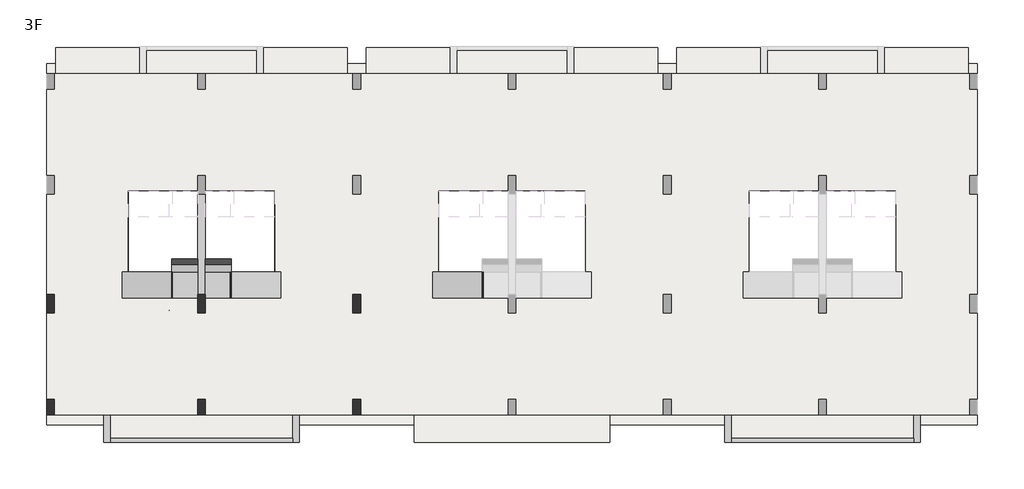
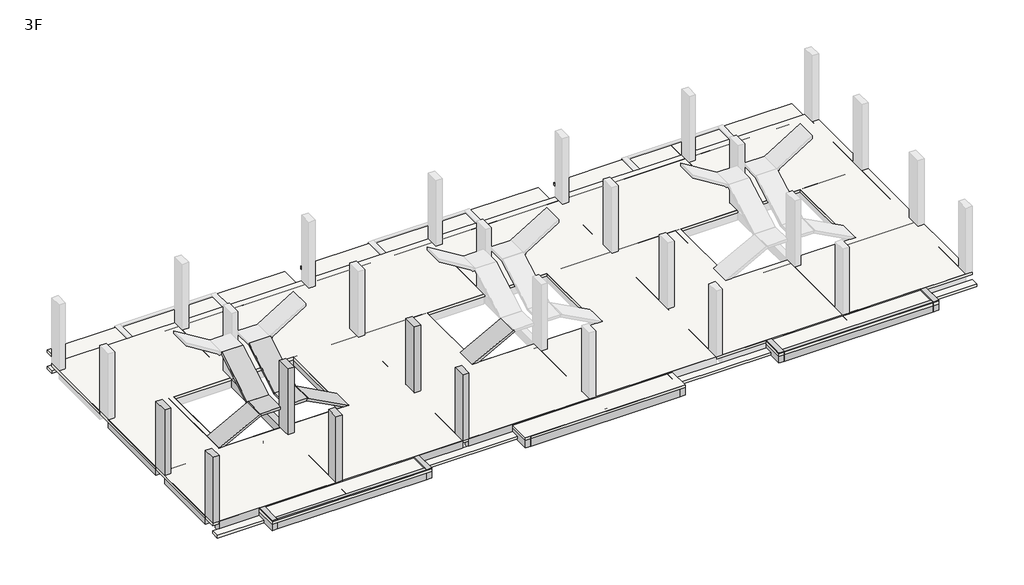
# One storey, part 1 of 3: 33 beams, 6 columns, 3 slabs.
"""IFC4 building model written with IfcOpenShell, lengths in millimetres."""

from ifc_helpers import new_model, si_unit, frame, origin, place, context, project, spatial, polyline, outline, extrude, faceted_brep, element, save

model = new_model("IFC4")

# Units and contexts
model_context = context("Model", 3, world=origin())
ifc_project = project(units=[si_unit("LENGTHUNIT", "METRE", prefix="MILLI")], contexts=[model_context])

# Site, building, storey
site = spatial("IfcSite", under=ifc_project)
building = spatial("IfcBuilding", under=site)
storey = spatial("IfcBuildingStorey", under=building, Name="3F", Elevation=7330.0)

# Beams
placement = place(None, origin())
element("IfcBeam", 1, ObjectType="M_Concrete-Rectangular Beam : 1000x120", at=placement, inside=storey, context=model_context, shape_type="Brep", body=[
    faceted_brep([(4730.4772067, 5424.9999998, 8380.0), (4730.4772067, 4424.9999998, 8380.0), (4787.1330577, 4424.9999998, 8274.2166623), (4787.1330577, 5424.9999998, 8274.2166623), (4700.0000007, 5424.9999998, 8363.6768996), (2770.0, 5424.9999998, 7330.0), (2770.0, 4424.9999998, 7330.0), (4700.0000007, 4424.9999998, 8363.6768996), (3024.1661582, 4424.9999998, 7330.0), (4760.5888269, 4424.9999998, 8260.0), (3024.1661582, 4449.9999998, 7330.0), (3020.0, 4449.9999998, 7327.7686728), (3020.0, 5424.9999998, 7327.7686728), (4760.5888269, 5424.9999998, 8260.0), (3020.0, 5424.9999998, 7330.0), (3020.0, 4449.9999998, 7330.0)], [[[0, 1, 2, 3]], [[1, 0, 4, 5, 6, 7]], [[2, 1, 7, 6, 8, 9]], [[3, 2, 9, 8, 10, 11, 12, 13]], [[0, 3, 13, 12, 14, 5, 4]], [[5, 14, 15, 10, 8, 6]], [[14, 12, 11, 15]], [[10, 15, 11]]]),
])
element("IfcBeam", 2, ObjectType="M_Concrete-Rectangular Beam : 1000x120", at=placement, inside=storey, context=model_context, shape_type="Brep", body=[
    faceted_brep([(4700.0000007, 7550.0000002, 9580.0), (5700.0000007, 7550.0000002, 9580.0), (5700.0000007, 7609.0063595, 9475.5095719), (4700.0000007, 7609.0063595, 9475.5095719), (4700.0000007, 5424.9999998, 8380.0), (4700.0000007, 5484.0063591, 8275.5095719), (5700.0000007, 5484.0063591, 8275.5095719), (5700.0000007, 5424.9999998, 8380.0), (5700.0000007, 5524.9999998, 8298.6589219), (5700.0000007, 7581.5414925, 9460.0), (4700.0000007, 5524.9999998, 8298.6589219), (4700.0000007, 7581.5414925, 9460.0)], [[[0, 1, 2, 3]], [[4, 5, 6, 7]], [[1, 0, 4, 7]], [[2, 1, 7, 6, 8, 9]], [[3, 2, 9, 8, 6, 5, 10, 11]], [[0, 3, 11, 10, 5, 4]]]),
])
element("IfcBeam", 3, ObjectType="M_Concrete-Rectangular Beam : 1000x120", at=placement, inside=storey, context=model_context, shape_type="Brep", body=[
    faceted_brep([(5700.0000007, 5524.9999998, 8260.0), (4700.0000007, 5524.9999998, 8260.0), (4700.0000007, 5524.9999998, 8298.6589219), (5700.0000007, 5524.9999998, 8298.6589219), (5700.0000007, 4424.9999998, 8260.0), (5700.0000007, 4424.9999998, 8380.0), (4730.4772067, 4424.9999998, 8380.0), (4787.1330577, 4424.9999998, 8274.2166623), (4760.5888269, 4424.9999998, 8260.0), (5700.0000007, 5424.9999998, 8380.0), (4700.0000007, 5424.9999998, 8380.0), (4700.0000007, 4424.9999998, 8380.0), (5700.0000007, 5484.0063591, 8275.5095719), (4760.5888269, 5424.9999998, 8260.0), (4700.0000007, 5424.9999998, 8260.0), (4700.0000007, 4424.9999998, 8363.6768996), (4700.0000007, 5484.0063591, 8275.5095719), (4700.0000007, 5424.9999998, 8363.6768996), (4730.4772067, 5424.9999998, 8380.0), (4787.1330577, 5424.9999998, 8274.2166623)], [[[0, 1, 2, 3]], [[4, 5, 6, 7, 8]], [[6, 5, 9, 10, 11]], [[5, 4, 0, 3, 12, 9]], [[1, 0, 4, 8, 13, 14]], [[15, 11, 10, 16, 2, 1, 14, 17]], [[6, 18, 19, 7]], [[18, 6, 15, 17]], [[7, 19, 13, 8]], [[19, 18, 17, 14, 13]], [[11, 15, 6]], [[12, 16, 10, 9]], [[16, 12, 3, 2]]]),
])
element("IfcBeam", 4, ObjectType="M_Concrete-Rectangular Beam : 1000x120", at=placement, inside=storey, context=model_context, shape_type="Brep", body=[
    faceted_brep([(6969.5227948, 4424.9999998, 8380.0), (6969.5227948, 5424.9999998, 8380.0), (6912.8669437, 5424.9999998, 8274.2166623), (6912.8669437, 4424.9999998, 8274.2166623), (7000.0000007, 4424.9999998, 8363.6768996), (8930.0000014, 4424.9999998, 7330.0), (8930.0000014, 5424.9999998, 7330.0), (7000.0000007, 5424.9999998, 8363.6768996), (6939.4111745, 4424.9999998, 8260.0), (8675.8338433, 4424.9999998, 7330.0), (6939.4111745, 5424.9999998, 8260.0), (8680.0, 5424.9999998, 7327.7686736), (8680.0, 4449.9999998, 7327.7686736), (8675.8338433, 4449.9999998, 7330.0), (8680.0, 5424.9999998, 7330.0), (8680.0, 4449.9999998, 7330.0)], [[[0, 1, 2, 3]], [[1, 0, 4, 5, 6, 7]], [[0, 3, 8, 9, 5, 4]], [[3, 2, 10, 11, 12, 13, 9, 8]], [[2, 1, 7, 6, 14, 11, 10]], [[9, 13, 15, 14, 6, 5]], [[11, 14, 15, 12]], [[15, 13, 12]]]),
])
element("IfcBeam", 5, ObjectType="M_Concrete-Rectangular Beam : 1000x120", at=placement, inside=storey, context=model_context, shape_type="Brep", body=[
    faceted_brep([(7000.0000007, 7550.0000002, 9580.0), (7000.0000007, 7609.0063595, 9475.5095719), (6000.0000007, 7609.0063595, 9475.5095719), (6000.0000007, 7550.0000002, 9580.0), (7000.0000007, 5424.9999998, 8380.0), (6000.0000007, 5424.9999998, 8380.0), (6000.0000007, 5484.0063591, 8275.5095719), (7000.0000007, 5484.0063591, 8275.5095719), (6000.0000007, 7581.5414925, 9460.0), (6000.0000007, 5524.9999998, 8298.6589219), (7000.0000007, 7581.5414925, 9460.0), (7000.0000007, 5524.9999998, 8298.6589219)], [[[0, 1, 2, 3]], [[4, 5, 6, 7]], [[3, 5, 4, 0]], [[2, 8, 9, 6, 5, 3]], [[1, 10, 11, 7, 6, 9, 8, 2]], [[0, 4, 7, 11, 10, 1]]]),
])
element("IfcBeam", 6, ObjectType="M_Concrete-Rectangular Beam : 1000x120", at=placement, inside=storey, context=model_context, shape_type="Brep", body=[
    faceted_brep([(7000.0000007, 5524.9999998, 8260.0), (6000.0000007, 5524.9999998, 8260.0), (6000.0000007, 5524.9999998, 8298.6589219), (7000.0000007, 5524.9999998, 8298.6589219), (6000.0000007, 4424.9999998, 8380.0), (6000.0000007, 4424.9999998, 8260.0), (6939.4111745, 4424.9999998, 8260.0), (6912.8669437, 4424.9999998, 8274.2166623), (6969.5227948, 4424.9999998, 8380.0), (7000.0000007, 4424.9999998, 8380.0), (7000.0000007, 5424.9999998, 8380.0), (6000.0000007, 5424.9999998, 8380.0), (6000.0000007, 5484.0063591, 8275.5095719), (7000.0000007, 5424.9999998, 8260.0), (6939.4111745, 5424.9999998, 8260.0), (7000.0000007, 4424.9999998, 8363.6768996), (7000.0000007, 5424.9999998, 8363.6768996), (7000.0000007, 5484.0063591, 8275.5095719), (6969.5227948, 5424.9999998, 8380.0), (6912.8669437, 5424.9999998, 8274.2166623)], [[[0, 1, 2, 3]], [[4, 5, 6, 7, 8]], [[8, 9, 10, 11, 4]], [[5, 4, 11, 12, 2, 1]], [[1, 0, 13, 14, 6, 5]], [[9, 15, 16, 13, 0, 3, 17, 10]], [[18, 8, 7, 19]], [[8, 18, 16, 15]], [[19, 7, 6, 14]], [[18, 19, 14, 13, 16]], [[15, 9, 8]], [[17, 12, 11, 10]], [[12, 17, 3, 2]]]),
])
element("IfcBeam", 7, ObjectType="M_Concrete-Rectangular Beam : 1000x120", at=placement, inside=storey, context=model_context, shape_type="Brep", body=[
    faceted_brep([(16730.4772117, 5424.9999998, 8380.0), (16730.4772117, 4424.9999998, 8380.0), (16787.1330628, 4424.9999998, 8274.2166623), (16787.1330628, 5424.9999998, 8274.2166623), (16700.0000058, 5424.9999998, 8363.6768996), (14770.000005, 5424.9999998, 7330.0), (14770.000005, 4424.9999998, 7330.0), (16700.0000058, 4424.9999998, 8363.6768996), (15024.1661632, 4424.9999998, 7330.0), (16760.588832, 4424.9999998, 8260.0), (15024.1661632, 4449.9999998, 7330.0), (15020.0000057, 4449.9999998, 7327.7686732), (15020.0000057, 5424.9999998, 7327.7686732), (16760.588832, 5424.9999998, 8260.0), (15020.0000057, 5424.9999998, 7330.0), (15020.0000057, 4449.9999998, 7330.0)], [[[0, 1, 2, 3]], [[1, 0, 4, 5, 6, 7]], [[2, 1, 7, 6, 8, 9]], [[3, 2, 9, 8, 10, 11, 12, 13]], [[0, 3, 13, 12, 14, 5, 4]], [[5, 14, 15, 10, 8, 6]], [[14, 12, 11, 15]], [[10, 15, 11]]]),
])
element("IfcBeam", 8, ObjectType="M_Concrete-Rectangular Beam : 150x500", at=placement, inside=storey, context=model_context, shape_type="SweptSolid", body=[
    extrude(outline(polyline([(2320.0000398, -1149.9999998), (2320.0000398, -999.9999998), (9380.0000399, -999.9999998), (9380.0000399, -1149.9999998), (2320.0000398, -1149.9999998)])), frame((0.0, 0.0, 6830.0), z_axis=(0.0, 0.0, 1.0), x_axis=(1.0, 0.0, 0.0)), (0.0, 0.0, 1.0), 500.0),
])
element("IfcBeam", 9, ObjectType="M_Concrete-Rectangular Beam : 150x500", at=placement, inside=storey, context=model_context, shape_type="SweptSolid", body=[
    extrude(outline(polyline([(26320.012858, -1150.2407813), (26320.012858, -1000.2407813), (33380.0128581, -1000.2407813), (33380.0128581, -1150.2407813), (26320.012858, -1150.2407813)])), frame((0.0, 0.0, 6830.0), z_axis=(0.0, 0.0, 1.0), x_axis=(1.0, 0.0, 0.0)), (0.0, 0.0, 1.0), 500.0),
])
element("IfcBeam", 10, ObjectType="M_Concrete-Rectangular Beam : 150x500", at=placement, inside=storey, context=model_context, shape_type="Brep", body=[
    faceted_brep([(14320.0998335, -1000.2407813, 7280.0), (14320.0998335, -1150.2407813, 7280.0), (21380.0998336, -1150.2407813, 7280.0), (21380.0998336, -1000.2407813, 7280.0), (18000.0064311, -1000.2407813, 7280.0), (17700.0064311, -1000.2407813, 7280.0), (14320.0998335, -1150.2407813, 6780.0), (21380.0998336, -1150.2407813, 6780.0), (14320.0998335, -1000.2407813, 6780.0), (21380.0998336, -1000.2407813, 6780.0)], [[[0, 1, 2, 3, 4, 5]], [[1, 6, 7, 2]], [[6, 8, 9, 7]], [[8, 0, 5, 4, 3, 9]], [[1, 0, 8, 6]], [[3, 2, 7, 9]]]),
])
element("IfcBeam", 11, ObjectType="M_Concrete-Rectangular Beam : 250x400", at=placement, inside=storey, context=model_context, shape_type="Brep", body=[
    faceted_brep([(8930.0, 8549.9999993, 7330.0), (8680.0, 8549.9999993, 7330.0), (8680.0, 5424.9999998, 7330.0), (8680.0, 4449.9999998, 7330.0), (8930.0, 4449.9999998, 7330.0), (8680.0, 8549.9999993, 7188.8582236), (8680.0, 8549.9999993, 6930.0), (8680.0, 4449.9999998, 6930.0), (8680.0, 4449.9999998, 7327.7686736), (8930.0, 8549.9999993, 6930.0), (8930.0, 4449.9999998, 6930.0)], [[[0, 1, 2, 3, 4]], [[1, 5, 6, 7, 8, 3, 2]], [[6, 9, 10, 7]], [[9, 0, 4, 10]], [[1, 0, 9, 6, 5]], [[4, 3, 8, 7, 10]]]),
])
element("IfcBeam", 12, ObjectType="M_Concrete-Rectangular Beam : 250x400", at=placement, inside=storey, context=model_context, shape_type="Brep", body=[
    faceted_brep([(3020.0, 8549.9999993, 7330.0), (2770.0, 8549.9999993, 7330.0), (2770.0, 4449.9999998, 7330.0), (3020.0, 4449.9999998, 7330.0), (3020.0, 5424.9999998, 7330.0), (3020.0, 8549.9999993, 6930.0), (3020.0, 8549.9999993, 7188.8582245), (3020.0, 4449.9999998, 7327.7686728), (3020.0, 4449.9999998, 6930.0), (2770.0, 8549.9999993, 6930.0), (2770.0, 4449.9999998, 6930.0)], [[[0, 1, 2, 3, 4]], [[5, 6, 0, 4, 3, 7, 8]], [[9, 5, 8, 10]], [[1, 9, 10, 2]], [[1, 0, 6, 5, 9]], [[3, 2, 10, 8, 7]]]),
])
element("IfcBeam", 13, ObjectType="M_Concrete-Rectangular Beam : 250x500", at=placement, inside=storey, context=model_context, shape_type="Brep", body=[
    faceted_brep([(2070.0000398, -1149.9999998, 7330.0), (2320.0000398, -1149.9999998, 7330.0), (2320.0000398, -999.9999998, 7330.0), (2320.0000398, -100.0000007, 7330.0), (2070.0000398, -100.0000007, 7330.0), (2320.0000398, -1149.9999998, 6830.0), (2320.0000398, -999.9999998, 6830.0), (2320.0000398, -100.0000007, 6830.0), (2070.0000398, -1149.9999998, 6830.0), (2070.0000398, -100.0000007, 6830.0)], [[[0, 1, 2, 3, 4]], [[1, 5, 6, 7, 3, 2]], [[5, 8, 9, 7, 6]], [[8, 0, 4, 9]], [[4, 3, 7, 9]], [[1, 0, 8, 5]]]),
])
element("IfcBeam", 14, ObjectType="M_Concrete-Rectangular Beam : 250x500", at=placement, inside=storey, context=model_context, shape_type="Brep", body=[
    faceted_brep([(9380.0000399, -1149.9999998, 7330.0), (9630.0000399, -1149.9999998, 7330.0), (9630.0000399, -100.0000007, 7330.0), (9380.0000399, -100.0000007, 7330.0), (9380.0000399, -999.9999998, 7330.0), (9380.0000399, -1149.9999998, 6830.0), (9380.0000399, -100.0000007, 6830.0), (9380.0000399, -999.9999998, 6830.0), (9630.0000399, -1149.9999998, 6830.0), (9630.0000399, -100.0000007, 6830.0)], [[[0, 1, 2, 3, 4]], [[5, 0, 4, 3, 6, 7]], [[8, 5, 7, 6, 9]], [[1, 8, 9, 2]], [[1, 0, 5, 8]], [[3, 2, 9, 6]]]),
])
element("IfcBeam", 15, ObjectType="M_Concrete-Rectangular Beam : 250x500", at=placement, inside=storey, context=model_context, shape_type="Brep", body=[
    faceted_brep([(26070.012858, -1150.2407813, 7330.0), (26320.012858, -1150.2407813, 7330.0), (26320.012858, -1000.2407813, 7330.0), (26320.012858, -97.7280146, 7330.0), (26070.012858, -97.7280146, 7330.0), (26320.012858, -1150.2407813, 6830.0), (26320.012858, -1000.2407813, 6830.0), (26320.012858, -97.7280146, 6830.0), (26070.012858, -1150.2407813, 6830.0), (26070.012858, -97.7280146, 6830.0)], [[[0, 1, 2, 3, 4]], [[1, 5, 6, 7, 3, 2]], [[5, 8, 9, 7, 6]], [[8, 0, 4, 9]], [[1, 0, 8, 5]], [[4, 3, 7, 9]]]),
])
element("IfcBeam", 16, ObjectType="M_Concrete-Rectangular Beam : 250x500", at=placement, inside=storey, context=model_context, shape_type="Brep", body=[
    faceted_brep([(33380.0128581, -1150.2407813, 7330.0), (33630.0128581, -1150.2407813, 7330.0), (33630.0128581, -97.7280146, 7330.0), (33380.0128581, -97.7280146, 7330.0), (33380.0128581, -1000.2407813, 7330.0), (33380.0128581, -1150.2407813, 6830.0), (33380.0128581, -97.7280146, 6830.0), (33380.0128581, -1000.2407813, 6830.0), (33630.0128581, -1150.2407813, 6830.0), (33630.0128581, -97.7280146, 6830.0)], [[[0, 1, 2, 3, 4]], [[5, 0, 4, 3, 6, 7]], [[8, 5, 7, 6, 9]], [[1, 8, 9, 2]], [[1, 0, 5, 8]], [[3, 2, 9, 6]]]),
])
element("IfcBeam", 17, ObjectType="M_Concrete-Rectangular Beam : 250x500", at=placement, inside=storey, context=model_context, shape_type="Brep", body=[
    faceted_brep([(14320.0998335, 149.9999992, 6780.0), (14070.0998335, 149.9999992, 6780.0), (14070.0998335, 149.9999992, 6830.0), (14320.0998335, 149.9999992, 6830.0), (14070.0998335, -1150.2407813, 7280.0), (14320.0998335, -1150.2407813, 7280.0), (14320.0998335, -1000.2407813, 7280.0), (14320.0998335, -100.0000007, 7280.0), (14070.0998335, -100.0000007, 7280.0), (14320.0998335, -1150.2407813, 6780.0), (14320.0998335, -1000.2407813, 6780.0), (14320.0998335, -100.0000007, 6830.0), (14070.0998335, -1150.2407813, 6780.0), (14070.0998335, -100.0000007, 6830.0)], [[[0, 1, 2, 3]], [[4, 5, 6, 7, 8]], [[9, 10, 0, 3, 11, 7, 6, 5]], [[1, 0, 10, 9, 12]], [[1, 12, 4, 8, 13, 2]], [[5, 4, 12, 9]], [[11, 13, 8, 7]], [[13, 11, 3, 2]]]),
])
element("IfcBeam", 18, ObjectType="M_Concrete-Rectangular Beam : 250x500", at=placement, inside=storey, context=model_context, shape_type="Brep", body=[
    faceted_brep([(21630.0998336, 149.9999992, 6780.0), (21380.0998336, 149.9999992, 6780.0), (21380.0998336, 149.9999992, 6830.0), (21630.0998336, 149.9999992, 6830.0), (21380.0998336, -1150.2407813, 7280.0), (21630.0998336, -1150.2407813, 7280.0), (21630.0998336, -100.0000007, 7280.0), (21380.0998336, -100.0000007, 7280.0), (21380.0998336, -1000.2407813, 7280.0), (21380.0998336, -1000.2407813, 6780.0), (21380.0998336, -1150.2407813, 6780.0), (21380.0998336, -100.0000007, 6830.0), (21630.0998336, -1150.2407813, 6780.0), (21630.0998336, -100.0000007, 6830.0)], [[[0, 1, 2, 3]], [[4, 5, 6, 7, 8]], [[1, 9, 10, 4, 8, 7, 11, 2]], [[1, 0, 12, 10, 9]], [[12, 0, 3, 13, 6, 5]], [[5, 4, 10, 12]], [[13, 11, 7, 6]], [[11, 13, 3, 2]]]),
])
element("IfcBeam", 19, ObjectType="M_Concrete-Rectangular Beam : 300x400", at=placement, inside=storey, context=model_context, shape_type="SweptSolid", body=[
    extrude(outline(polyline([(165.0, 4550.0000002), (-135.0, 4550.0000002), (-135.0, 8449.9985388), (165.0, 8449.9985388), (165.0, 4550.0000002)])), frame((0.0, 0.0, 6930.0), z_axis=(0.0, 0.0, 1.0), x_axis=(1.0, 0.0, 0.0)), (0.0, 0.0, 1.0), 400.0),
])
element("IfcBeam", 20, ObjectType="M_Concrete-Rectangular Beam : 300x400", at=placement, inside=storey, context=model_context, shape_type="SweptSolid", body=[
    extrude(outline(polyline([(165.0, 499.9999998), (-135.0, 499.9999998), (-135.0, 3850.0000002), (165.0, 3850.0000002), (165.0, 499.9999998)])), frame((0.0, 0.0, 6930.0), z_axis=(0.0, 0.0, 1.0), x_axis=(1.0, 0.0, 0.0)), (0.0, 0.0, 1.0), 400.0),
])
element("IfcBeam", 21, ObjectType="M_Concrete-Rectangular Beam : 300x400", at=placement, inside=storey, context=model_context, shape_type="SweptSolid", body=[
    extrude(outline(polyline([(12000.0000027, 4550.0000002), (11700.0000027, 4550.0000002), (11700.0000027, 8449.9985388), (12000.0000027, 8449.9985388), (12000.0000027, 4550.0000002)])), frame((0.0, 0.0, 6930.0), z_axis=(0.0, 0.0, 1.0), x_axis=(1.0, 0.0, 0.0)), (0.0, 0.0, 1.0), 400.0),
])
element("IfcBeam", 22, ObjectType="M_Concrete-Rectangular Beam : 300x400", at=placement, inside=storey, context=model_context, shape_type="SweptSolid", body=[
    extrude(outline(polyline([(6000.0, 4550.0000002), (5700.0, 4550.0000002), (5700.0, 8449.9985388), (6000.0, 8449.9985388), (6000.0, 4550.0000002)])), frame((0.0, 0.0, 6930.0), z_axis=(0.0, 0.0, 1.0), x_axis=(1.0, 0.0, 0.0)), (0.0, 0.0, 1.0), 400.0),
])
element("IfcBeam", 23, ObjectType="M_Concrete-Rectangular Beam : 300x400", at=placement, inside=storey, context=model_context, shape_type="SweptSolid", body=[
    extrude(outline(polyline([(6000.0000007, 499.9999998), (5700.0000007, 499.9999998), (5700.0000007, 3850.0000002), (6000.0000007, 3850.0000002), (6000.0000007, 499.9999998)])), frame((0.0, 0.0, 6930.0), z_axis=(0.0, 0.0, 1.0), x_axis=(1.0, 0.0, 0.0)), (0.0, 0.0, 1.0), 400.0),
])
element("IfcBeam", 24, ObjectType="M_Concrete-Rectangular Beam : 300x400", at=placement, inside=storey, context=model_context, shape_type="SweptSolid", body=[
    extrude(outline(polyline([(12000.0000034, 499.9999998), (11700.0000034, 499.9999998), (11700.0000034, 3850.0000002), (12000.0000034, 3850.0000002), (12000.0000034, 499.9999998)])), frame((0.0, 0.0, 6930.0), z_axis=(0.0, 0.0, 1.0), x_axis=(1.0, 0.0, 0.0)), (0.0, 0.0, 1.0), 400.0),
])
element("IfcBeam", 25, ObjectType="M_Concrete-Rectangular Beam : 300x400", at=placement, inside=storey, context=model_context, shape_type="Brep", body=[
    faceted_brep([(6000.0000007, -100.0000002, 7280.0), (5700.0000007, -100.0000007, 7280.0), (5700.0000007, -999.9999998, 7280.0), (6000.0000007, -999.9999998, 7280.0), (6000.0000007, -100.0000002, 6880.0), (6000.0000007, -999.9999998, 6880.0), (5700.0000007, -100.0000007, 6880.0), (5700.0000007, -999.9999998, 6880.0)], [[[0, 1, 2, 3]], [[4, 0, 3, 5]], [[6, 4, 5, 7]], [[1, 6, 7, 2]], [[6, 1, 0, 4]], [[3, 2, 7, 5]]]),
])
element("IfcBeam", 26, ObjectType="M_Concrete-Rectangular Beam : 300x400", at=placement, inside=storey, context=model_context, shape_type="Brep", body=[
    faceted_brep([(18000.0064311, -1000.2407813, 7280.0), (17700.0064311, -1000.2407813, 7280.0), (17700.0064311, -1000.2407813, 6880.0), (18000.0064311, -1000.2407813, 6880.0), (18000.0064311, -100.0000002, 7280.0), (17700.0064311, -100.0000007, 7280.0), (18000.0064311, -100.0000002, 6880.0), (17700.0064311, -100.0000007, 6880.0)], [[[0, 1, 2, 3]], [[1, 0, 4, 5]], [[0, 3, 6, 4]], [[3, 2, 7, 6]], [[2, 1, 5, 7]], [[4, 6, 7, 5]]]),
])
element("IfcBeam", 27, ObjectType="M_Concrete-Rectangular Beam : 300x400", at=placement, inside=storey, context=model_context, shape_type="SweptSolid", body=[
    extrude(outline(polyline([(29700.0064292, -100.0000002), (30000.0064292, -100.0000002), (30000.0064292, -1000.2407813), (29700.0064292, -1000.2407813), (29700.0064292, -100.0000002)])), frame((0.0, 0.0, 6880.0), z_axis=(0.0, 0.0, 1.0), x_axis=(1.0, 0.0, 0.0)), (0.0, 0.0, 1.0), 400.0),
])
element("IfcBeam", 28, ObjectType="M_Concrete-Rectangular Beam : 300x500", at=placement, inside=storey, context=model_context, shape_type="Brep", body=[
    faceted_brep([(165.0, 4449.9999998, 7330.0), (165.0, 4149.9999998, 7330.0), (5700.0000007, 4149.9999998, 7330.0), (5700.0000007, 4449.9999998, 7330.0), (3024.1661582, 4449.9999998, 7330.0), (3020.0, 4449.9999998, 7330.0), (2770.0, 4449.9999998, 7330.0), (165.0, 4149.9999998, 6830.0), (5700.0000007, 4149.9999998, 6830.0), (165.0, 4449.9999998, 6830.0), (5700.0000007, 4449.9999998, 6830.0)], [[[0, 1, 2, 3, 4, 5, 6]], [[1, 7, 8, 2]], [[7, 9, 10, 8]], [[9, 0, 6, 5, 4, 3, 10]], [[1, 0, 9, 7]], [[3, 2, 8, 10]]]),
])
element("IfcBeam", 29, ObjectType="M_Concrete-Rectangular Beam : 300x500", at=placement, inside=storey, context=model_context, shape_type="Brep", body=[
    faceted_brep([(165.0, 199.9999993, 7330.0), (165.0, -100.0000007, 7330.0), (2070.0000398, -100.0000007, 7330.0), (2320.0000398, -100.0000007, 7330.0), (5700.0000007, -100.0000007, 7330.0), (5700.0000007, 199.9999993, 7330.0), (165.0, -100.0000007, 6830.0), (2070.0000398, -100.0000007, 6830.0), (2320.0000398, -100.0000007, 6830.0), (5700.0000007, -100.0000007, 6830.0), (165.0, 199.9999993, 6830.0), (5700.0000007, 199.9999993, 6830.0)], [[[0, 1, 2, 3, 4, 5]], [[1, 6, 7, 8, 9, 4, 3, 2]], [[6, 10, 11, 9, 8, 7]], [[10, 0, 5, 11]], [[1, 0, 10, 6]], [[5, 4, 9, 11]]]),
])
element("IfcBeam", 30, ObjectType="M_Concrete-Rectangular Beam : 300x500", at=placement, inside=storey, context=model_context, shape_type="Brep", body=[
    faceted_brep([(6000.0000007, 4449.9999998, 7330.0), (6000.0000007, 4149.9999998, 7330.0), (11700.0000034, 4149.9999998, 7330.0), (11700.0000034, 4449.9999998, 7330.0), (8930.0, 4449.9999998, 7330.0), (8680.0, 4449.9999998, 7330.0), (8675.8338433, 4449.9999998, 7330.0), (6000.0000007, 4149.9999998, 6830.0), (11700.0000034, 4149.9999998, 6830.0), (6000.0000007, 4449.9999998, 6830.0), (11700.0000034, 4449.9999998, 6830.0)], [[[0, 1, 2, 3, 4, 5, 6]], [[1, 7, 8, 2]], [[7, 9, 10, 8]], [[9, 0, 6, 5, 4, 3, 10]], [[1, 0, 9, 7]], [[3, 2, 8, 10]]]),
])
element("IfcBeam", 31, ObjectType="M_Concrete-Rectangular Beam : 300x500", at=placement, inside=storey, context=model_context, shape_type="Brep", body=[
    faceted_brep([(6000.0000007, 199.9999993, 7330.0), (6000.0000007, -100.0000007, 7330.0), (9380.0000399, -100.0000007, 7330.0), (9630.0000399, -100.0000007, 7330.0), (11700.0000034, -100.0000007, 7330.0), (11700.0000034, 199.9999993, 7330.0), (6000.0000007, -100.0000007, 6830.0), (9380.0000399, -100.0000007, 6830.0), (9630.0000399, -100.0000007, 6830.0), (11700.0000034, -100.0000007, 6830.0), (6000.0000007, 199.9999993, 6830.0), (11700.0000034, 199.9999993, 6830.0)], [[[0, 1, 2, 3, 4, 5]], [[1, 6, 7, 8, 9, 4, 3, 2]], [[6, 10, 11, 9, 8, 7]], [[10, 0, 5, 11]], [[1, 0, 10, 6]], [[5, 4, 9, 11]]]),
])
element("IfcBeam", 32, ObjectType="M_Concrete-Rectangular Beam : 300x500", at=placement, inside=storey, context=model_context, shape_type="Brep", body=[
    faceted_brep([(12000.0000027, 4449.9999998, 7330.0), (12000.0000034, 4149.9999998, 7330.0), (17700.0000058, 4149.9999998, 7330.0), (17700.0000058, 4449.9999998, 7330.0), (15024.1661632, 4449.9999998, 7330.0), (15020.0000057, 4449.9999998, 7330.0), (14770.0000057, 4449.9999998, 7330.0), (12000.0000034, 4149.9999998, 6830.0), (17700.0000058, 4149.9999998, 6830.0), (12000.0000034, 4449.9999998, 6830.0), (17700.0000058, 4449.9999998, 6830.0)], [[[0, 1, 2, 3, 4, 5, 6]], [[1, 7, 8, 2]], [[7, 9, 10, 8]], [[9, 0, 6, 5, 4, 3, 10]], [[7, 1, 0, 9]], [[3, 2, 8, 10]]]),
])
element("IfcBeam", 33, ObjectType="M_Concrete-Rectangular Beam : 300x500", at=placement, inside=storey, context=model_context, shape_type="Brep", body=[
    faceted_brep([(12000.0000034, 199.9999993, 7330.0), (12000.0000034, -100.0000007, 7330.0), (17700.0000058, -100.0000007, 7330.0), (17700.0000058, 199.9999993, 7330.0), (12000.0000034, -100.0000007, 6830.0), (14070.0998335, -100.0000007, 6830.0), (14320.0998335, -100.0000007, 6830.0), (17700.0000058, -100.0000007, 6830.0), (12000.0000034, 199.9999993, 6830.0), (17700.0000058, 199.9999993, 6830.0)], [[[0, 1, 2, 3]], [[1, 4, 5, 6, 7, 2]], [[4, 8, 9, 7, 6, 5]], [[8, 0, 3, 9]], [[4, 1, 0, 8]], [[3, 2, 7, 9]]]),
])

# Columns
element("IfcColumn", 34, ObjectType="M_Concrete-Rectangular-Column : 300x600", at=placement, inside=storey, context=model_context, shape_type="SweptSolid", body=[
    extrude(outline(polyline([(165.0, 500.0), (165.0, -100.0), (-135.0, -100.0), (-135.0, 500.0), (165.0, 500.0)])), frame((0.0, 0.0, 7330.0), z_axis=(0.0, 0.0, 1.0), x_axis=(1.0, 0.0, 0.0)), (0.0, 0.0, 1.0), 3300.0),
])
element("IfcColumn", 35, ObjectType="M_Concrete-Rectangular-Column : 300x600", at=placement, inside=storey, context=model_context, shape_type="SweptSolid", body=[
    extrude(outline(polyline([(6000.0000007, 500.0), (6000.0000007, -100.0), (5700.0000007, -100.0), (5700.0000007, 500.0), (6000.0000007, 500.0)])), frame((0.0, 0.0, 7330.0), z_axis=(0.0, 0.0, 1.0), x_axis=(1.0, 0.0, 0.0)), (0.0, 0.0, 1.0), 3300.0),
])
element("IfcColumn", 36, ObjectType="M_Concrete-Rectangular-Column : 300x600", at=placement, inside=storey, context=model_context, shape_type="SweptSolid", body=[
    extrude(outline(polyline([(12000.0000034, 500.0), (12000.0000034, -100.0), (11700.0000034, -100.0), (11700.0000034, 500.0), (12000.0000034, 500.0)])), frame((0.0, 0.0, 7330.0), z_axis=(0.0, 0.0, 1.0), x_axis=(1.0, 0.0, 0.0)), (0.0, 0.0, 1.0), 3300.0),
])
element("IfcColumn", 37, ObjectType="M_Concrete-Rectangular-Column : 300x700", at=placement, inside=storey, context=model_context, shape_type="SweptSolid", body=[
    extrude(outline(polyline([(165.0, 4550.0000002), (165.0, 3850.0000002), (-135.0, 3850.0000002), (-135.0, 4550.0000002), (165.0, 4550.0000002)])), frame((0.0, 0.0, 7330.0), z_axis=(0.0, 0.0, 1.0), x_axis=(1.0, 0.0, 0.0)), (0.0, 0.0, 1.0), 3300.0),
])
element("IfcColumn", 38, ObjectType="M_Concrete-Rectangular-Column : 300x700", at=placement, inside=storey, context=model_context, shape_type="SweptSolid", body=[
    extrude(outline(polyline([(6000.0000007, 4550.0000002), (6000.0000007, 3850.0000002), (5700.0000007, 3850.0000002), (5700.0000007, 4550.0000002), (6000.0000007, 4550.0000002)])), frame((0.0, 0.0, 7330.0), z_axis=(0.0, 0.0, 1.0), x_axis=(1.0, 0.0, 0.0)), (0.0, 0.0, 1.0), 3300.0),
])
element("IfcColumn", 39, ObjectType="M_Concrete-Rectangular-Column : 300x700", at=placement, inside=storey, context=model_context, shape_type="SweptSolid", body=[
    extrude(outline(polyline([(12000.0000034, 4550.0000002), (12000.0000034, 3850.0000002), (11700.0000034, 3850.0000002), (11700.0000034, 4550.0000002), (12000.0000034, 4550.0000002)])), frame((0.0, 0.0, 7330.0), z_axis=(0.0, 0.0, 1.0), x_axis=(1.0, 0.0, 0.0)), (0.0, 0.0, 1.0), 3300.0),
])

# Slabs
element("IfcSlab", 40, ObjectType="130", at=placement, inside=storey, context=model_context, shape_type="SweptSolid", body=[
    extrude(outline(polyline([(35835.035019, 13100.0000001), (35835.035019, -97.7280146), (-135.0, -97.7280146), (-135.0, 13100.0000001), (35835.035019, 13100.0000001)]), holes=[polyline([(8680.0, 4450.0000002), (8680.0, 8549.9999993), (3020.0, 8549.9999993), (3020.0, 4450.0000002), (8680.0, 4450.0000002)]), polyline([(20680.0000058, 8549.9999993), (15020.0000057, 8549.9999993), (15020.0000057, 4449.9992702), (20680.0000058, 4449.9992702), (20680.0000058, 8549.9999993)]), polyline([(32680.0000108, 8549.9999993), (27020.000004, 8549.9999993), (27020.000004, 4449.9999998), (32680.0000108, 4449.9999998), (32680.0000108, 8549.9999993)])]), frame((0.0, 0.0, 7200.0), z_axis=(0.0, 0.0, 1.0), x_axis=(1.0, 0.0, 0.0)), (0.0, 0.0, 1.0), 130.0),
])
element("IfcSlab", 41, ObjectType="130", at=placement, inside=storey, context=model_context, shape_type="SweptSolid", body=[
    extrude(outline(polyline([(26070.012858, -1150.2407813), (26070.012858, -97.7280146), (33630.0128581, -97.7280146), (33630.0128581, -1150.2407813), (26070.012858, -1150.2407813)])), frame((0.0, 0.0, 7150.0), z_axis=(0.0, 0.0, 1.0), x_axis=(1.0, 0.0, 0.0)), (0.0, 0.0, 1.0), 130.0),
    extrude(outline(polyline([(14070.0998335, -1150.2407813), (14070.0998335, -100.0000007), (21630.0998336, -100.0000007), (21630.0998336, -1150.2407813), (14070.0998335, -1150.2407813)])), frame((0.0, 0.0, 7150.0), z_axis=(0.0, 0.0, 1.0), x_axis=(1.0, 0.0, 0.0)), (0.0, 0.0, 1.0), 130.0),
    extrude(outline(polyline([(2070.0000398, -1149.9999998), (2070.0000398, -100.0000003), (9630.0000399, -100.0000003), (9630.0000399, -1149.9999998), (2070.0000398, -1149.9999998)])), frame((0.0, 0.0, 7150.0), z_axis=(0.0, 0.0, 1.0), x_axis=(1.0, 0.0, 0.0)), (0.0, 0.0, 1.0), 130.0),
    extrude(outline(polyline([(225.0000002, 13100.0000001), (225.0000002, 14100.0000002), (3459.9999747, 14100.0000002), (3459.9999747, 14150.0000066), (8240.0000277, 14150.0000066), (8240.0000277, 14100.0000002), (11474.9871465, 14100.0000002), (11474.9871465, 13100.0000001), (225.0000002, 13100.0000001)])), frame((0.0, 0.0, 7150.0), z_axis=(0.0, 0.0, 1.0), x_axis=(1.0, 0.0, 0.0)), (0.0, 0.0, 1.0), 130.0),
    extrude(outline(polyline([(12225.349842, 13100.0000001), (12225.349842, 14100.0000002), (15460.0998466, 14100.0000002), (15460.0998466, 14150.0000066), (20239.9825383, 14150.0000066), (20239.9825383, 14100.0000002), (23474.8705392, 14100.0000002), (23474.8705392, 13100.0000001), (12225.349842, 13100.0000001)])), frame((0.0, 0.0, 7150.0), z_axis=(0.0, 0.0, 1.0), x_axis=(1.0, 0.0, 0.0)), (0.0, 0.0, 1.0), 130.0),
    extrude(outline(polyline([(24225.0128576, 13100.0000001), (24225.0128576, 14100.0000002), (27460.0128711, 14100.0000002), (27460.0128711, 14150.0000066), (32239.900241, 14150.0000066), (32239.900241, 14100.0000002), (35474.516002, 14100.0000002), (35474.516002, 13100.0000001), (24225.0128576, 13100.0000001)])), frame((0.0, 0.0, 7150.0), z_axis=(0.0, 0.0, 1.0), x_axis=(1.0, 0.0, 0.0)), (0.0, 0.0, 1.0), 130.0),
])
element("IfcSlab", 42, ObjectType="130", at=placement, inside=storey, context=model_context, shape_type="SweptSolid", body=[
    extrude(outline(polyline([(12225.349842, 13485.0000009), (12225.349842, 13100.0000001), (11474.9999626, 13100.0000001), (11474.9999626, 13485.0000009), (12225.349842, 13485.0000009)])), frame((0.0, 0.0, 6830.0), z_axis=(0.0, 0.0, 1.0), x_axis=(1.0, 0.0, 0.0)), (0.0, 0.0, 1.0), 130.0),
    extrude(outline(polyline([(24225.000042, 13485.0000009), (24225.000042, 13101.5853605), (23474.9999676, 13101.5853605), (23474.9999676, 13485.0000009), (24225.000042, 13485.0000009)])), frame((0.0, 0.0, 6830.0), z_axis=(0.0, 0.0, 1.0), x_axis=(1.0, 0.0, 0.0)), (0.0, 0.0, 1.0), 130.0),
    extrude(outline(polyline([(35835.035019, 13485.0000009), (35835.035019, 13100.0000001), (35474.9999657, 13100.0000001), (35474.9999657, 13485.0000009), (35835.035019, 13485.0000009)])), frame((0.0, 0.0, 6830.0), z_axis=(0.0, 0.0, 1.0), x_axis=(1.0, 0.0, 0.0)), (0.0, 0.0, 1.0), 130.0),
    extrude(outline(polyline([(35834.7667691, -97.7280146), (35834.7667691, -484.9999998), (33630.0128581, -484.9999998), (33630.0128581, -97.7280146), (35834.7667691, -97.7280146)])), frame((0.0, 0.0, 6830.0), z_axis=(0.0, 0.0, 1.0), x_axis=(1.0, 0.0, 0.0)), (0.0, 0.0, 1.0), 130.0),
    extrude(outline(polyline([(26070.012858, -100.0000007), (26070.012858, -485.2422366), (21630.0998336, -485.2422366), (21630.0998336, -100.0000007), (26070.012858, -100.0000007)])), frame((0.0, 0.0, 6830.0), z_axis=(0.0, 0.0, 1.0), x_axis=(1.0, 0.0, 0.0)), (0.0, 0.0, 1.0), 130.0),
    extrude(outline(polyline([(14070.0998335, -100.0000003), (14070.0998335, -484.9918007), (9630.0000399, -484.9918007), (9630.0000399, -100.0000003), (14070.0998335, -100.0000003)])), frame((0.0, 0.0, 6830.0), z_axis=(0.0, 0.0, 1.0), x_axis=(1.0, 0.0, 0.0)), (0.0, 0.0, 1.0), 130.0),
    extrude(outline(polyline([(2070.0000398, -100.0000002), (2070.0000398, -484.9999998), (-135.0, -484.9999998), (-135.0, -100.0000002), (2070.0000398, -100.0000002)])), frame((0.0, 0.0, 6830.0), z_axis=(0.0, 0.0, 1.0), x_axis=(1.0, 0.0, 0.0)), (0.0, 0.0, 1.0), 130.0),
    extrude(outline(polyline([(225.0000398, 13485.0000009), (225.0000398, 13101.5853605), (-134.9299604, 13101.5853605), (-134.9299604, 13485.0000009), (225.0000398, 13485.0000009)])), frame((0.0, 0.0, 6830.0), z_axis=(0.0, 0.0, 1.0), x_axis=(1.0, 0.0, 0.0)), (0.0, 0.0, 1.0), 130.0),
])

save(model, "model.ifc")

# Revit data of these elements
# Type "M_Concrete-Rectangular Beam : 1000x120"
#   Length [instance default] = 1524 mm
#   b = 1000 mm
#   h = 120 mm
#   Structural Material [instance default] = Concrete, Cast-in-Place gray
#   Assembly Code = ""
# Type "M_Concrete-Rectangular Beam : 150x500"
#   Length [instance default] = 1524 mm
#   b = 150 mm
#   h = 500 mm
#   Structural Material [instance default] = Concrete, Cast-in-Place gray
#   Assembly Code = ""
# Type "M_Concrete-Rectangular Beam : 250x400"
#   Length [instance default] = 1524 mm
#   b = 250 mm
#   h = 400 mm
#   Structural Material [instance default] = Concrete, Cast-in-Place gray
#   Assembly Code = ""
# Type "M_Concrete-Rectangular Beam : 250x500"
#   Length [instance default] = 1524 mm
#   b = 250 mm
#   h = 500 mm
#   Structural Material [instance default] = Concrete, Cast-in-Place gray
#   Assembly Code = ""
# Type "M_Concrete-Rectangular Beam : 300x400"
#   Length [instance default] = 1524 mm
#   b = 300 mm
#   h = 400 mm
#   Structural Material [instance default] = Concrete, Cast-in-Place gray
#   Assembly Code = ""
# Type "M_Concrete-Rectangular Beam : 300x500"
#   Length [instance default] = 1524 mm
#   b = 300 mm
#   h = 500 mm
#   Structural Material [instance default] = Concrete, Cast-in-Place gray
#   Assembly Code = ""
# Type "M_Concrete-Rectangular-Column : 300x600"
#   b = 300 mm
#   h = 600 mm
#   Structural Material [instance default] = Concrete, Cast-in-Place gray
# Type "M_Concrete-Rectangular-Column : 300x700"
#   b = 300 mm
#   h = 700 mm
#   Structural Material [instance default] = Concrete, Cast-in-Place gray
# Type "130"
#   Function = 0
#   Layers, outside or top first: 130 mm "VM.TM1A-Concrete Wall-M250" (function 1)
# Elements 1, 4, 7 (IfcBeam, "M_Concrete-Rectangular Beam : 1000x120")
#   Comments = ""
#   COF_GEN__Name = "STAIR"
#   Structural Material = Concrete, Cast-in-Place gray
#   Phase Created = New Construction
#   Materials on its faces: "Concrete, Cast-in-Place gray"
# Elements 2, 3, 5, 6 (IfcBeam, "M_Concrete-Rectangular Beam : 1000x120")
#   COF_GEN__Name = "STAIR"
#   Structural Material = Concrete, Cast-in-Place gray
#   Phase Created = New Construction
#   Materials on its faces: "Concrete, Cast-in-Place gray"
# Elements 8, 9, 10 (IfcBeam, "M_Concrete-Rectangular Beam : 150x500")
#   Comments = ""
#   COF_CON__WorkItemNumber = "SH3-A-03F"
#   COF_GEN__Name = "DP4"
#   Structural Material = Concrete, Cast-in-Place gray
#   Phase Created = New Construction
#   Materials on its faces: "Concrete, Cast-in-Place gray"
# Elements 11, 12 (IfcBeam, "M_Concrete-Rectangular Beam : 250x400")
#   Comments = ""
#   COF_CON__WorkItemNumber = "SH3-A-03F"
#   COF_GEN__Name = "DP1"
#   Structural Material = Concrete, Cast-in-Place gray
#   Phase Created = New Construction
#   Materials on its faces: "Concrete, Cast-in-Place gray"
# Elements 13, 14, 15, 16, 17, 18 (IfcBeam, "M_Concrete-Rectangular Beam : 250x500")
#   Comments = ""
#   COF_CON__WorkItemNumber = "SH3-A-03F"
#   COF_GEN__Name = "DP2"
#   Structural Material = Concrete, Cast-in-Place gray
#   Phase Created = New Construction
#   Materials on its faces: "Concrete, Cast-in-Place gray"
# Elements 19, 20, 21, 24 (IfcBeam, "M_Concrete-Rectangular Beam : 300x400")
#   Comments = ""
#   COF_CON__WorkItemNumber = "SH3-A-03F"
#   COF_GEN__Name = "D3"
#   Structural Material = Concrete, Cast-in-Place gray
#   Phase Created = New Construction
#   Materials on its faces: "Concrete, Cast-in-Place gray"
# Elements 22, 23, 25, 26, 27 (IfcBeam, "M_Concrete-Rectangular Beam : 300x400")
#   Comments = ""
#   COF_CON__WorkItemNumber = "SH3-A-03F"
#   COF_GEN__Name = "D5"
#   Structural Material = Concrete, Cast-in-Place gray
#   Phase Created = New Construction
#   Materials on its faces: "Concrete, Cast-in-Place gray"
# Elements 28, 30, 32 (IfcBeam, "M_Concrete-Rectangular Beam : 300x500")
#   Comments = ""
#   COF_CON__WorkItemNumber = "SH3-A-03F"
#   COF_GEN__Name = "D2"
#   Structural Material = Concrete, Cast-in-Place gray
#   Phase Created = New Construction
#   Materials on its faces: "Concrete, Cast-in-Place gray"
# Elements 29, 31, 33 (IfcBeam, "M_Concrete-Rectangular Beam : 300x500")
#   Comments = ""
#   COF_CON__WorkItemNumber = "SH3-A-03F"
#   COF_GEN__Name = "D1"
#   Structural Material = Concrete, Cast-in-Place gray
#   Phase Created = New Construction
#   Materials on its faces: "Concrete, Cast-in-Place gray"
# Elements 34, 35, 36 (IfcColumn, "M_Concrete-Rectangular-Column : 300x600")
#   Comments = ""
#   COF_CON__WorkItemNumber = "SH3-A-04F"
#   COF_GEN__Name = "C1"
#   Structural Material = Concrete, Cast-in-Place gray
#   Phase Created = New Construction
#   Materials on its faces: "Concrete, Cast-in-Place gray"
# Element 37 (IfcColumn, "M_Concrete-Rectangular-Column : 300x700")
#   Comments = ""
#   COF_CON__WorkItemNumber = "SH3-A-04F"
#   COF_GEN__Name = "C3"
#   Structural Material = Concrete, Cast-in-Place gray
#   Phase Created = New Construction
#   Materials on its faces: "Concrete, Cast-in-Place gray"
# Element 38 (IfcColumn, "M_Concrete-Rectangular-Column : 300x700")
#   Comments = ""
#   COF_CON__WorkItemNumber = "SH3-A-04F"
#   COF_GEN__Name = "C4"
#   Structural Material = Concrete, Cast-in-Place gray
#   Phase Created = New Construction
#   Materials on its faces: "Concrete, Cast-in-Place gray"
# Element 39 (IfcColumn, "M_Concrete-Rectangular-Column : 300x700")
#   Comments = ""
#   COF_CON__WorkItemNumber = "SH3-A-04F"
#   COF_GEN__Name = "C5"
#   Structural Material = Concrete, Cast-in-Place gray
#   Phase Created = New Construction
#   Materials on its faces: "Concrete, Cast-in-Place gray"
# Element 40 (IfcSlab, "130")
#   COF_CON__WorkItemNumber = "SH3-A-03F"
#   COF_GEN__Name = "T130"
#   Height Offset From Level = 0 mm
#   Phase Created = New Construction
#   Materials on its faces: "VM.TM1A-Concrete Wall-M250"
# Element 41 (IfcSlab, "130")
#   COF_CON__WorkItemNumber = "SH3-A-03F"
#   COF_GEN__Name = "T130"
#   Height Offset From Level = -50 mm
#   Phase Created = New Construction
#   Materials on its faces: "VM.TM1A-Concrete Wall-M250"
# Element 42 (IfcSlab, "130")
#   COF_GEN__Name = "T130"
#   Height Offset From Level = -370 mm
#   Phase Created = New Construction
#   Materials on its faces: "VM.TM1A-Concrete Wall-M250"
# Materials
#   "Concrete, Cast-in-Place gray": class "Concrete", colour RGB 207 208 204, transparency 0, Description = "Cast-in-place concrete", Cost = 0
#   "VM.TM1A-Concrete Wall-M250": class "Concrete", colour RGB 192 192 192, transparency 0, Description = "Cast-in-place concrete", Cost = 0
